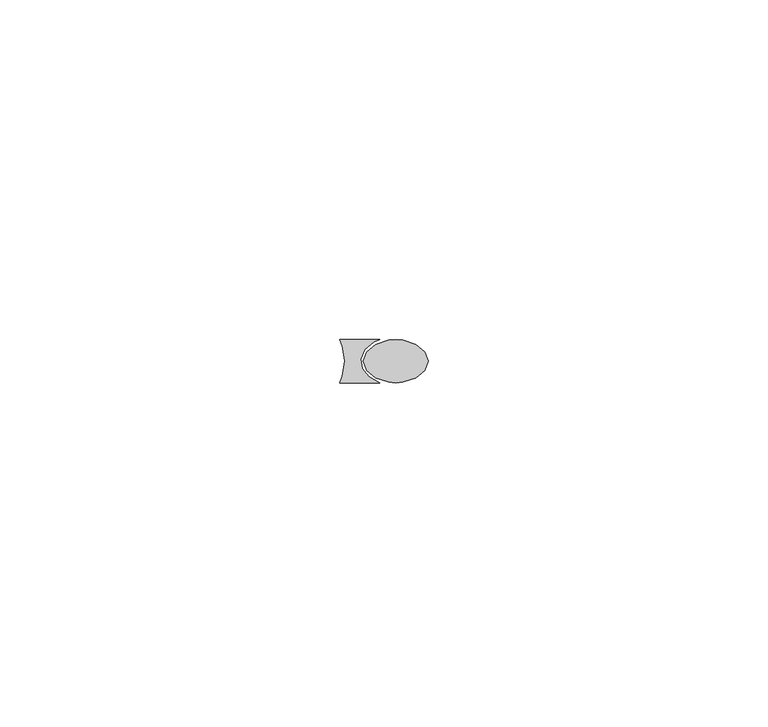
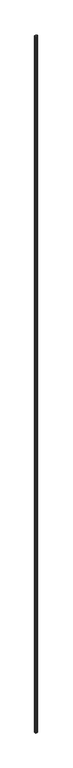
"""IFC4 building model written with IfcOpenShell, lengths in millimetres: proxy geometry, Generic Models 11:Generic Models 1:306267:Generic Models 1:306267 : Generic Models 11:Generic Models 1:306267:300405:Generic Models 1:306267:Generic Models 1:306267 : Generic Models 11:Generic Models 1:306267:300405 : Generic Models 11:Generic Models 1:306267:Generic Models 1:306267 : Generic Models 11:Generic Models 1:306267:300405:9 : Generic Models 11:Generic Models 1:306267:Generic Models 1:306267 : Generic Models 11:Generic Models 1:306267:300405:Generic Models 1:306267:Generic Models 1:306267 : Generic Models 11:Generic Models 1:306267:300405 : Generic Models 11:Generic Models 1:306267:Generic Models 1:306267 : Generic Models 11:Generic Models 1:306267:300405:300182."""

from ifc_helpers import new_model, si_unit, origin, origin_with_axes, place, context, project, spatial, polyline, outline, extrude, source, transform, mapped, element, save


def generic_models_35decbb9(model_context):
    return source(origin(), model_context, "Body", "SweptSolid", [
        extrude(outline(polyline([(570437.5275794, -578999.3138032), (570438.8490734, -578998.2090691), (570440.7586877, -578997.595988), (570441.8184436, -578997.5163841), (570442.8781996, -578997.595988), (570444.7878138, -578998.2090691), (570446.1093078, -578999.3138032), (570446.5809436, -579000.6913841), (570446.1093078, -579002.068965), (570444.7878138, -579003.173699), (570442.8781996, -579003.7867802), (570441.8184436, -579003.8663841), (570440.7586877, -579003.7867802), (570438.8490734, -579003.173699), (570437.5275794, -579002.068965), (570437.0559436, -579000.6913841), (570437.5275794, -578999.3138032)])), origin_with_axes(), (0.0, 0.0, 1.0), 3695.7),
        extrude(outline(polyline([(570433.9641325, -579002.9006209), (570434.2778186, -579000.6913841), (570433.9641325, -578998.4821473), (570433.5867239, -578997.5163841), (570439.454816, -578997.5163841), (570438.5945351, -578997.9027017), (570437.2849599, -578998.9861871), (570436.6846064, -579000.3364349), (570436.8873943, -579001.7422111), (570437.8615993, -579002.9835952), (570439.454816, -579003.8663841), (570433.5867239, -579003.8663841), (570433.9641325, -579002.9006209)])), origin_with_axes(), (0.0, 0.0, 1.0), 3695.7),
    ])


if __name__ == "__main__":
    model = new_model("IFC4")
    model_context = context("Model", 3, world=origin())
    ifc_project = project(units=[si_unit("LENGTHUNIT", "METRE", prefix="MILLI")], contexts=[model_context])
    site = spatial("IfcSite", under=ifc_project)
    building = spatial("IfcBuilding", under=site)
    placement = place(None, origin())
    generic_models_shape = generic_models_35decbb9(model_context)
    element("IfcBuildingElementProxy", 1, Name="Generic Models 11:Generic Models 1:306267:Generic Models 1:306267 : Generic Models 11:Generic Models 1:306267:300405:Generic Models 1:306267:Generic Models 1:306267 : Generic Models 11:Generic Models 1:306267:300405 : Generic Models 11:Generic Models 1:306267:Generic Models 1:306267 : Generic Models 11:Generic Models 1:306267:300405:9 : Generic Models 11:Generic Models 1:306267:Generic Models 1:306267 : Generic Models 11:Generic Models 1:306267:300405:Generic Models 1:306267:Generic Models 1:306267 : Generic Models 11:Generic Models 1:306267:300405 : Generic Models 11:Generic Models 1:306267:Generic Models 1:306267 : Generic Models 11:Generic Models 1:306267:300405:300182", ObjectType="Generic Models 11:Generic Models 1:306267:Generic Models 1:306267 : Generic Models 11:Generic Models 1:306267:300405:Generic Models 1:306267:Generic Models 1:306267 : Generic Models 11:Generic Models 1:306267:300405 : Generic Models 11:Generic Models 1:306267:Generic Models 1:306267 : Generic Models 11:Generic Models 1:306267:300405:9 : Generic Models 11:Generic Models 1:306267:Generic Models 1:306267 : Generic Models 11:Generic Models 1:306267:300405:Generic Models 1:306267:Generic Models 1:306267 : Generic Models 11:Generic Models 1:306267:300405 : Generic Models 11:Generic Models 1:306267:Generic Models 1:306267 : Generic Models 11:Generic Models 1:306267:300405:300182", at=placement, inside=building, context=model_context, shape_type="MappedRepresentation", body=[
        mapped(generic_models_shape, transform((0.0, 0.0, 0.0), x_axis=(1.0, 0.0, 0.0), y_axis=(0.0, 1.0, 0.0), z_axis=(0.0, 0.0, 1.0))),
    ])
    save(model, "model.ifc")

# Revit data of these elements
# Type "Generic Models 11:Generic Models 1:306267:Generic Models 1:306267 : Generic Models 11:Generic Models 1:306267:300405:Generic Models 1:306267:Generic Models 1:306267 : Generic Models 11:Generic Models 1:306267:300405 : Generic Models 11:Generic Models 1:306267:Generic Models 1:306267 : Generic Models 11:Generic Models 1:306267:300405:9 : Generic Models 11:Generic Models 1:306267:Generic Models 1:306267 : Generic Models 11:Generic Models 1:306267:300405:Generic Models 1:306267:Generic Models 1:306267 : Generic Models 11:Generic Models 1:306267:300405 : Generic Models 11:Generic Models 1:306267:Generic Models 1:306267 : Generic Models 11:Generic Models 1:306267:300405:300182"
#   NameOverride = "Generic Models 11:Generic Models 1:306267:Generic Models 1:306267 : Generic Models 11:Generic Models 1:306267:300405:Generic Models 1:306267:Generic Models 1:306267 : Generic Models 11:Generic Models 1:306267:300405 : Generic Models 11:Generic Models 1:306267:Generic Models 1:306267 : Generic Models 11:Generic Models 1:306267:300405:300182"
#   ObjectTypeOverride = "Generic Models 1:306267:Generic Models 1:306267 : Generic Models 11:Generic Models 1:306267:300405 : Generic Models 11:Generic Models 1:306267:Generic Models 1:306267 : Generic Models 11:Generic Models 1:306267:300405"
#   Reference = "Generic Models 1"
#   Tag = "300182"
# Element 1 (IfcBuildingElementProxy, "Generic Models 11:Generic Models 1:306267:Generic Models 1:306267 : Generic Models 11:Generic Models 1:306267:300405:Generic Models 1:306267:Generic Models 1:306267 : Generic Models 11:Generic Models 1:306267:300405 : Generic Models 11:Generic Models 1:306267:Generic Models 1:306267 : Generic Models 11:Generic Models 1:306267:300405:9 : Generic Models 11:Generic Models 1:306267:Generic Models 1:306267 : Generic Models 11:Generic Models 1:306267:300405:Generic Models 1:306267:Generic Models 1:306267 : Generic Models 11:Generic Models 1:306267:300405 : Generic Models 11:Generic Models 1:306267:Generic Models 1:306267 : Generic Models 11:Generic Models 1:306267:300405:300182")
#   Materials on its faces: "SEALANT & BACKER ROD, IF NECESSARY"
# Materials
#   "SEALANT & BACKER ROD, IF NECESSARY": class "Unassigned", colour RGB 120 120 120, transparency 0, Cost = 0
